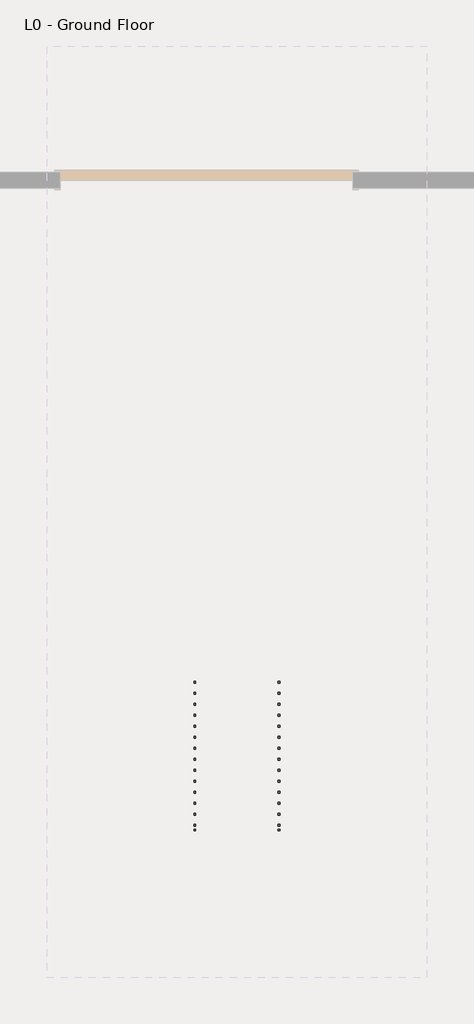
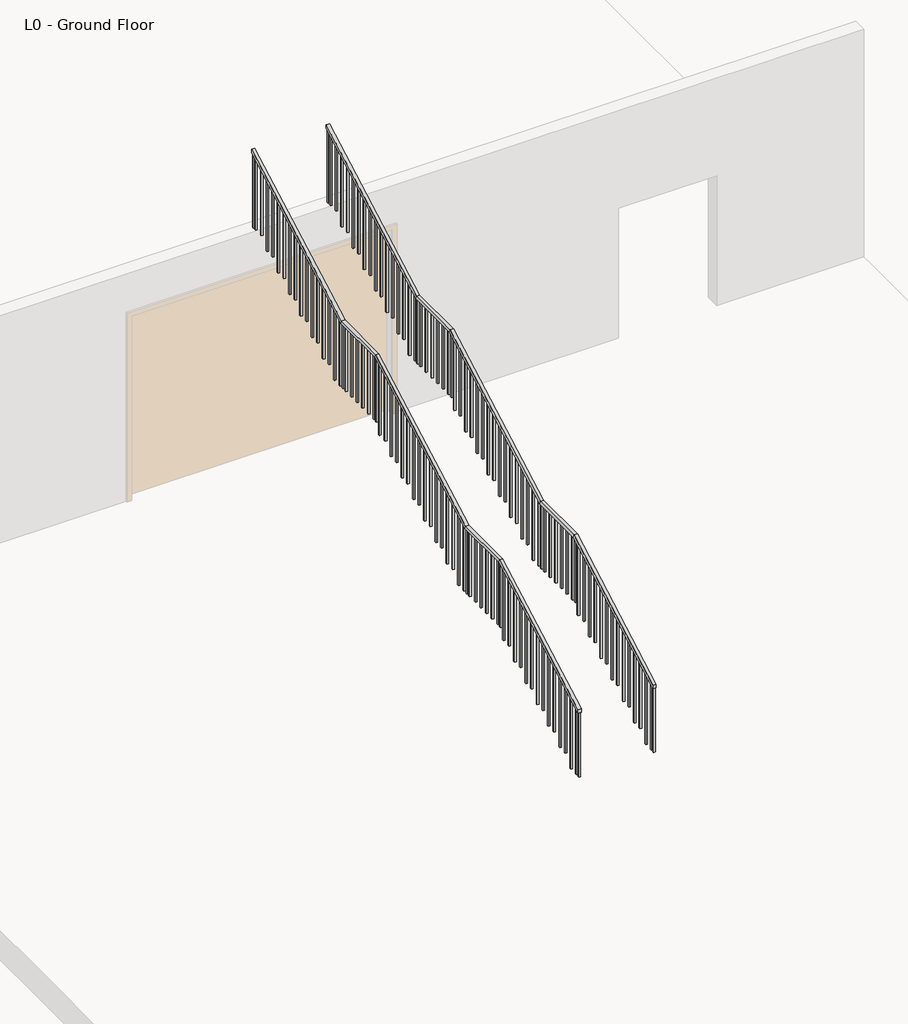
# One storey, part 10 of 14: 2 railings.
"""IFC4 building model written with IfcOpenShell, lengths in millimetres."""

from ifc_helpers import new_model, si_unit, frame, origin, place, context, project, spatial, polyline, outline, extrude, faceted_brep, element, save

model = new_model("IFC4")

# Units and contexts
model_context = context("Model", 3, world=origin())
ifc_project = project(units=[si_unit("LENGTHUNIT", "METRE", prefix="MILLI")], contexts=[model_context])

# Site, building, storey
site = spatial("IfcSite", under=ifc_project)
building = spatial("IfcBuilding", under=site)
storey = spatial("IfcBuildingStorey", under=building, Name="L0 - Ground Floor", Elevation=0.0)

# Railings
placement = place(None, origin())
element("IfcRailing", 1, ObjectType="1100mm", at=placement, inside=storey, context=model_context, shape_type="SolidModel", body=[
    faceted_brep([(20443.6510627, -13941.7341454, 1266.6666667), (20443.6510627, -13941.7341454, 1209.4687214), (20493.6510627, -13941.7341454, 1209.4687214), (20493.6510627, -13941.7341454, 1266.6666667), (20443.6510627, -11841.7341454, 2433.3333333), (20443.6510627, -11828.7778439, 2383.3333333), (20493.6510627, -11828.7778439, 2383.3333333), (20493.6510627, -11841.7341454, 2433.3333333), (20443.6510627, -10941.7341454, 2433.3333333), (20443.6510627, -10928.7778439, 2383.3333333), (20493.6510627, -10928.7778439, 2383.3333333), (20493.6510627, -10941.7341454, 2433.3333333), (20443.6510627, -8541.7341454, 3766.6666667), (20443.6510627, -8528.7778439, 3716.6666667), (20493.6510627, -8528.7778439, 3716.6666667), (20493.6510627, -8541.7341454, 3766.6666667), (20443.6510627, -7641.7341454, 3766.6666667), (20443.6510627, -7628.7778439, 3716.6666667), (20493.6510627, -7628.7778439, 3716.6666667), (20493.6510627, -7641.7341454, 3766.6666667), (20443.6510627, -5241.7341454, 5100.0), (20493.6510627, -5241.7341454, 5100.0), (20493.6510627, -5241.7341454, 5042.8020548), (20443.6510627, -5241.7341454, 5042.8020548)], [[[0, 1, 2, 3]], [[1, 0, 4, 5]], [[2, 1, 5, 6]], [[3, 2, 6, 7]], [[0, 3, 7, 4]], [[5, 4, 8, 9]], [[6, 5, 9, 10]], [[7, 6, 10, 11]], [[4, 7, 11, 8]], [[9, 8, 12, 13]], [[10, 9, 13, 14]], [[11, 10, 14, 15]], [[8, 11, 15, 12]], [[13, 12, 16, 17]], [[14, 13, 17, 18]], [[15, 14, 18, 19]], [[12, 15, 19, 16]], [[20, 21, 22, 23]], [[17, 16, 20, 23]], [[18, 17, 23, 22]], [[19, 18, 22, 21]], [[16, 19, 21, 20]]]),
    extrude(outline(polyline([(-5329.2341454, 3833.3333333), (-5329.2341454, 4994.1909437), (-5304.2341454, 5008.0798326), (-5304.2341454, 3833.3333333), (-5329.2341454, 3833.3333333)])), frame((20456.1510627, 0.0, 0.0), z_axis=(1.0, 0.0, 0.0), x_axis=(0.0, 1.0, 0.0)), (0.0, 0.0, 1.0), 25.0),
    extrude(outline(polyline([(-5479.2341454, 3833.3333333), (-5479.2341454, 4910.8576103), (-5454.2341454, 4924.7464992), (-5454.2341454, 3833.3333333), (-5479.2341454, 3833.3333333)])), frame((20456.1510627, 0.0, 0.0), z_axis=(1.0, 0.0, 0.0), x_axis=(0.0, 1.0, 0.0)), (0.0, 0.0, 1.0), 25.0),
    extrude(outline(polyline([(-5629.2341454, 3666.6666667), (-5629.2341454, 4827.524277), (-5604.2341454, 4841.4131659), (-5604.2341454, 3666.6666667), (-5629.2341454, 3666.6666667)])), frame((20456.1510627, 0.0, 0.0), z_axis=(1.0, 0.0, 0.0), x_axis=(0.0, 1.0, 0.0)), (0.0, 0.0, 1.0), 25.0),
    extrude(outline(polyline([(-5779.2341454, 3666.6666667), (-5779.2341454, 4744.1909437), (-5754.2341454, 4758.0798326), (-5754.2341454, 3666.6666667), (-5779.2341454, 3666.6666667)])), frame((20456.1510627, 0.0, 0.0), z_axis=(1.0, 0.0, 0.0), x_axis=(0.0, 1.0, 0.0)), (0.0, 0.0, 1.0), 25.0),
    extrude(outline(polyline([(-5929.2341454, 3500.0), (-5929.2341454, 4660.8576103), (-5904.2341454, 4674.7464992), (-5904.2341454, 3500.0), (-5929.2341454, 3500.0)])), frame((20456.1510627, 0.0, 0.0), z_axis=(1.0, 0.0, 0.0), x_axis=(0.0, 1.0, 0.0)), (0.0, 0.0, 1.0), 25.0),
    extrude(outline(polyline([(-6079.2341454, 3500.0), (-6079.2341454, 4577.524277), (-6054.2341454, 4591.4131659), (-6054.2341454, 3500.0), (-6079.2341454, 3500.0)])), frame((20456.1510627, 0.0, 0.0), z_axis=(1.0, 0.0, 0.0), x_axis=(0.0, 1.0, 0.0)), (0.0, 0.0, 1.0), 25.0),
    extrude(outline(polyline([(-6229.2341454, 3333.3333333), (-6229.2341454, 4494.1909437), (-6204.2341454, 4508.0798326), (-6204.2341454, 3333.3333333), (-6229.2341454, 3333.3333333)])), frame((20456.1510627, 0.0, 0.0), z_axis=(1.0, 0.0, 0.0), x_axis=(0.0, 1.0, 0.0)), (0.0, 0.0, 1.0), 25.0),
    extrude(outline(polyline([(-6379.2341454, 3333.3333333), (-6379.2341454, 4410.8576103), (-6354.2341454, 4424.7464992), (-6354.2341454, 3333.3333333), (-6379.2341454, 3333.3333333)])), frame((20456.1510627, 0.0, 0.0), z_axis=(1.0, 0.0, 0.0), x_axis=(0.0, 1.0, 0.0)), (0.0, 0.0, 1.0), 25.0),
    extrude(outline(polyline([(-6529.2341454, 3166.6666667), (-6529.2341454, 4327.524277), (-6504.2341454, 4341.4131659), (-6504.2341454, 3166.6666667), (-6529.2341454, 3166.6666667)])), frame((20456.1510627, 0.0, 0.0), z_axis=(1.0, 0.0, 0.0), x_axis=(0.0, 1.0, 0.0)), (0.0, 0.0, 1.0), 25.0),
    extrude(outline(polyline([(-6679.2341454, 3166.6666667), (-6679.2341454, 4244.1909437), (-6654.2341454, 4258.0798326), (-6654.2341454, 3166.6666667), (-6679.2341454, 3166.6666667)])), frame((20456.1510627, 0.0, 0.0), z_axis=(1.0, 0.0, 0.0), x_axis=(0.0, 1.0, 0.0)), (0.0, 0.0, 1.0), 25.0),
    extrude(outline(polyline([(-6829.2341454, 3000.0), (-6829.2341454, 4160.8576103), (-6804.2341454, 4174.7464992), (-6804.2341454, 3000.0), (-6829.2341454, 3000.0)])), frame((20456.1510627, 0.0, 0.0), z_axis=(1.0, 0.0, 0.0), x_axis=(0.0, 1.0, 0.0)), (0.0, 0.0, 1.0), 25.0),
    extrude(outline(polyline([(-6979.2341454, 3000.0), (-6979.2341454, 4077.524277), (-6954.2341454, 4091.4131659), (-6954.2341454, 3000.0), (-6979.2341454, 3000.0)])), frame((20456.1510627, 0.0, 0.0), z_axis=(1.0, 0.0, 0.0), x_axis=(0.0, 1.0, 0.0)), (0.0, 0.0, 1.0), 25.0),
    extrude(outline(polyline([(-7129.2341454, 2833.3333333), (-7129.2341454, 3994.1909437), (-7104.2341454, 4008.0798326), (-7104.2341454, 2833.3333333), (-7129.2341454, 2833.3333333)])), frame((20456.1510627, 0.0, 0.0), z_axis=(1.0, 0.0, 0.0), x_axis=(0.0, 1.0, 0.0)), (0.0, 0.0, 1.0), 25.0),
    extrude(outline(polyline([(-7279.2341454, 2833.3333333), (-7279.2341454, 3910.8576103), (-7254.2341454, 3924.7464992), (-7254.2341454, 2833.3333333), (-7279.2341454, 2833.3333333)])), frame((20456.1510627, 0.0, 0.0), z_axis=(1.0, 0.0, 0.0), x_axis=(0.0, 1.0, 0.0)), (0.0, 0.0, 1.0), 25.0),
    extrude(outline(polyline([(-7429.2341454, 2666.6666667), (-7429.2341454, 3827.524277), (-7404.2341454, 3841.4131659), (-7404.2341454, 2666.6666667), (-7429.2341454, 2666.6666667)])), frame((20456.1510627, 0.0, 0.0), z_axis=(1.0, 0.0, 0.0), x_axis=(0.0, 1.0, 0.0)), (0.0, 0.0, 1.0), 25.0),
    extrude(outline(polyline([(-7579.2341454, 2666.6666667), (-7579.2341454, 3744.1909437), (-7554.2341454, 3758.0798326), (-7554.2341454, 2666.6666667), (-7579.2341454, 2666.6666667)])), frame((20456.1510627, 0.0, 0.0), z_axis=(1.0, 0.0, 0.0), x_axis=(0.0, 1.0, 0.0)), (0.0, 0.0, 1.0), 25.0),
    extrude(outline(polyline([(20481.1510627, -7729.2341454), (20456.1510627, -7729.2341454), (20456.1510627, -7704.2341454), (20481.1510627, -7704.2341454), (20481.1510627, -7729.2341454)])), frame((0.0, 0.0, 2666.6666667), z_axis=(0.0, 0.0, 1.0), x_axis=(1.0, 0.0, 0.0)), (0.0, 0.0, 1.0), 1050.0),
    extrude(outline(polyline([(20481.1510627, -7879.2341454), (20456.1510627, -7879.2341454), (20456.1510627, -7854.2341454), (20481.1510627, -7854.2341454), (20481.1510627, -7879.2341454)])), frame((0.0, 0.0, 2666.6666667), z_axis=(0.0, 0.0, 1.0), x_axis=(1.0, 0.0, 0.0)), (0.0, 0.0, 1.0), 1050.0),
    extrude(outline(polyline([(20481.1510627, -8029.2341454), (20456.1510627, -8029.2341454), (20456.1510627, -8004.2341454), (20481.1510627, -8004.2341454), (20481.1510627, -8029.2341454)])), frame((0.0, 0.0, 2666.6666667), z_axis=(0.0, 0.0, 1.0), x_axis=(1.0, 0.0, 0.0)), (0.0, 0.0, 1.0), 1050.0),
    extrude(outline(polyline([(20481.1510627, -8179.2341454), (20456.1510627, -8179.2341454), (20456.1510627, -8154.2341454), (20481.1510627, -8154.2341454), (20481.1510627, -8179.2341454)])), frame((0.0, 0.0, 2666.6666667), z_axis=(0.0, 0.0, 1.0), x_axis=(1.0, 0.0, 0.0)), (0.0, 0.0, 1.0), 1050.0),
    extrude(outline(polyline([(20481.1510627, -8329.2341454), (20456.1510627, -8329.2341454), (20456.1510627, -8304.2341454), (20481.1510627, -8304.2341454), (20481.1510627, -8329.2341454)])), frame((0.0, 0.0, 2666.6666667), z_axis=(0.0, 0.0, 1.0), x_axis=(1.0, 0.0, 0.0)), (0.0, 0.0, 1.0), 1050.0),
    extrude(outline(polyline([(20481.1510627, -8479.2341454), (20456.1510627, -8479.2341454), (20456.1510627, -8454.2341454), (20481.1510627, -8454.2341454), (20481.1510627, -8479.2341454)])), frame((0.0, 0.0, 2666.6666667), z_axis=(0.0, 0.0, 1.0), x_axis=(1.0, 0.0, 0.0)), (0.0, 0.0, 1.0), 1050.0),
    extrude(outline(polyline([(-8629.2341454, 2500.0), (-8629.2341454, 3660.8576103), (-8604.2341454, 3674.7464992), (-8604.2341454, 2500.0), (-8629.2341454, 2500.0)])), frame((20456.1510627, 0.0, 0.0), z_axis=(1.0, 0.0, 0.0), x_axis=(0.0, 1.0, 0.0)), (0.0, 0.0, 1.0), 25.0),
    extrude(outline(polyline([(-8779.2341454, 2500.0), (-8779.2341454, 3577.524277), (-8754.2341454, 3591.4131659), (-8754.2341454, 2500.0), (-8779.2341454, 2500.0)])), frame((20456.1510627, 0.0, 0.0), z_axis=(1.0, 0.0, 0.0), x_axis=(0.0, 1.0, 0.0)), (0.0, 0.0, 1.0), 25.0),
    extrude(outline(polyline([(-8929.2341454, 2333.3333333), (-8929.2341454, 3494.1909437), (-8904.2341454, 3508.0798326), (-8904.2341454, 2333.3333333), (-8929.2341454, 2333.3333333)])), frame((20456.1510627, 0.0, 0.0), z_axis=(1.0, 0.0, 0.0), x_axis=(0.0, 1.0, 0.0)), (0.0, 0.0, 1.0), 25.0),
    extrude(outline(polyline([(-9079.2341454, 2333.3333333), (-9079.2341454, 3410.8576103), (-9054.2341454, 3424.7464992), (-9054.2341454, 2333.3333333), (-9079.2341454, 2333.3333333)])), frame((20456.1510627, 0.0, 0.0), z_axis=(1.0, 0.0, 0.0), x_axis=(0.0, 1.0, 0.0)), (0.0, 0.0, 1.0), 25.0),
    extrude(outline(polyline([(-9229.2341454, 2166.6666667), (-9229.2341454, 3327.524277), (-9204.2341454, 3341.4131659), (-9204.2341454, 2166.6666667), (-9229.2341454, 2166.6666667)])), frame((20456.1510627, 0.0, 0.0), z_axis=(1.0, 0.0, 0.0), x_axis=(0.0, 1.0, 0.0)), (0.0, 0.0, 1.0), 25.0),
    extrude(outline(polyline([(-9379.2341454, 2166.6666667), (-9379.2341454, 3244.1909437), (-9354.2341454, 3258.0798326), (-9354.2341454, 2166.6666667), (-9379.2341454, 2166.6666667)])), frame((20456.1510627, 0.0, 0.0), z_axis=(1.0, 0.0, 0.0), x_axis=(0.0, 1.0, 0.0)), (0.0, 0.0, 1.0), 25.0),
    extrude(outline(polyline([(-9529.2341454, 2000.0), (-9529.2341454, 3160.8576103), (-9504.2341454, 3174.7464992), (-9504.2341454, 2000.0), (-9529.2341454, 2000.0)])), frame((20456.1510627, 0.0, 0.0), z_axis=(1.0, 0.0, 0.0), x_axis=(0.0, 1.0, 0.0)), (0.0, 0.0, 1.0), 25.0),
    extrude(outline(polyline([(-9679.2341454, 2000.0), (-9679.2341454, 3077.524277), (-9654.2341454, 3091.4131659), (-9654.2341454, 2000.0), (-9679.2341454, 2000.0)])), frame((20456.1510627, 0.0, 0.0), z_axis=(1.0, 0.0, 0.0), x_axis=(0.0, 1.0, 0.0)), (0.0, 0.0, 1.0), 25.0),
    extrude(outline(polyline([(-9829.2341454, 1833.3333333), (-9829.2341454, 2994.1909437), (-9804.2341454, 3008.0798326), (-9804.2341454, 1833.3333333), (-9829.2341454, 1833.3333333)])), frame((20456.1510627, 0.0, 0.0), z_axis=(1.0, 0.0, 0.0), x_axis=(0.0, 1.0, 0.0)), (0.0, 0.0, 1.0), 25.0),
    extrude(outline(polyline([(-9979.2341454, 1833.3333333), (-9979.2341454, 2910.8576103), (-9954.2341454, 2924.7464992), (-9954.2341454, 1833.3333333), (-9979.2341454, 1833.3333333)])), frame((20456.1510627, 0.0, 0.0), z_axis=(1.0, 0.0, 0.0), x_axis=(0.0, 1.0, 0.0)), (0.0, 0.0, 1.0), 25.0),
    extrude(outline(polyline([(-10129.2341454, 1666.6666667), (-10129.2341454, 2827.524277), (-10104.2341454, 2841.4131659), (-10104.2341454, 1666.6666667), (-10129.2341454, 1666.6666667)])), frame((20456.1510627, 0.0, 0.0), z_axis=(1.0, 0.0, 0.0), x_axis=(0.0, 1.0, 0.0)), (0.0, 0.0, 1.0), 25.0),
    extrude(outline(polyline([(-10279.2341454, 1666.6666667), (-10279.2341454, 2744.1909437), (-10254.2341454, 2758.0798326), (-10254.2341454, 1666.6666667), (-10279.2341454, 1666.6666667)])), frame((20456.1510627, 0.0, 0.0), z_axis=(1.0, 0.0, 0.0), x_axis=(0.0, 1.0, 0.0)), (0.0, 0.0, 1.0), 25.0),
    extrude(outline(polyline([(-10429.2341454, 1500.0), (-10429.2341454, 2660.8576103), (-10404.2341454, 2674.7464992), (-10404.2341454, 1500.0), (-10429.2341454, 1500.0)])), frame((20456.1510627, 0.0, 0.0), z_axis=(1.0, 0.0, 0.0), x_axis=(0.0, 1.0, 0.0)), (0.0, 0.0, 1.0), 25.0),
    extrude(outline(polyline([(-10579.2341454, 1500.0), (-10579.2341454, 2577.524277), (-10554.2341454, 2591.4131659), (-10554.2341454, 1500.0), (-10579.2341454, 1500.0)])), frame((20456.1510627, 0.0, 0.0), z_axis=(1.0, 0.0, 0.0), x_axis=(0.0, 1.0, 0.0)), (0.0, 0.0, 1.0), 25.0),
    extrude(outline(polyline([(-10729.2341454, 1333.3333333), (-10729.2341454, 2494.1909437), (-10704.2341454, 2508.0798326), (-10704.2341454, 1333.3333333), (-10729.2341454, 1333.3333333)])), frame((20456.1510627, 0.0, 0.0), z_axis=(1.0, 0.0, 0.0), x_axis=(0.0, 1.0, 0.0)), (0.0, 0.0, 1.0), 25.0),
    extrude(outline(polyline([(-10879.2341454, 1333.3333333), (-10879.2341454, 2410.8576103), (-10854.2341454, 2424.7464992), (-10854.2341454, 1333.3333333), (-10879.2341454, 1333.3333333)])), frame((20456.1510627, 0.0, 0.0), z_axis=(1.0, 0.0, 0.0), x_axis=(0.0, 1.0, 0.0)), (0.0, 0.0, 1.0), 25.0),
    extrude(outline(polyline([(20481.1510627, -11029.2341454), (20456.1510627, -11029.2341454), (20456.1510627, -11004.2341454), (20481.1510627, -11004.2341454), (20481.1510627, -11029.2341454)])), frame((0.0, 0.0, 1333.3333333), z_axis=(0.0, 0.0, 1.0), x_axis=(1.0, 0.0, 0.0)), (0.0, 0.0, 1.0), 1050.0),
    extrude(outline(polyline([(20481.1510627, -11179.2341454), (20456.1510627, -11179.2341454), (20456.1510627, -11154.2341454), (20481.1510627, -11154.2341454), (20481.1510627, -11179.2341454)])), frame((0.0, 0.0, 1333.3333333), z_axis=(0.0, 0.0, 1.0), x_axis=(1.0, 0.0, 0.0)), (0.0, 0.0, 1.0), 1050.0),
    extrude(outline(polyline([(20481.1510627, -11329.2341454), (20456.1510627, -11329.2341454), (20456.1510627, -11304.2341454), (20481.1510627, -11304.2341454), (20481.1510627, -11329.2341454)])), frame((0.0, 0.0, 1333.3333333), z_axis=(0.0, 0.0, 1.0), x_axis=(1.0, 0.0, 0.0)), (0.0, 0.0, 1.0), 1050.0),
    extrude(outline(polyline([(20481.1510627, -11479.2341454), (20456.1510627, -11479.2341454), (20456.1510627, -11454.2341454), (20481.1510627, -11454.2341454), (20481.1510627, -11479.2341454)])), frame((0.0, 0.0, 1333.3333333), z_axis=(0.0, 0.0, 1.0), x_axis=(1.0, 0.0, 0.0)), (0.0, 0.0, 1.0), 1050.0),
    extrude(outline(polyline([(20481.1510627, -11629.2341454), (20456.1510627, -11629.2341454), (20456.1510627, -11604.2341454), (20481.1510627, -11604.2341454), (20481.1510627, -11629.2341454)])), frame((0.0, 0.0, 1333.3333333), z_axis=(0.0, 0.0, 1.0), x_axis=(1.0, 0.0, 0.0)), (0.0, 0.0, 1.0), 1050.0),
    extrude(outline(polyline([(20481.1510627, -11779.2341454), (20456.1510627, -11779.2341454), (20456.1510627, -11754.2341454), (20481.1510627, -11754.2341454), (20481.1510627, -11779.2341454)])), frame((0.0, 0.0, 1333.3333333), z_axis=(0.0, 0.0, 1.0), x_axis=(1.0, 0.0, 0.0)), (0.0, 0.0, 1.0), 1050.0),
    extrude(outline(polyline([(-11929.2341454, 1166.6666667), (-11929.2341454, 2327.524277), (-11904.2341454, 2341.4131659), (-11904.2341454, 1166.6666667), (-11929.2341454, 1166.6666667)])), frame((20456.1510627, 0.0, 0.0), z_axis=(1.0, 0.0, 0.0), x_axis=(0.0, 1.0, 0.0)), (0.0, 0.0, 1.0), 25.0),
    extrude(outline(polyline([(-12079.2341454, 1166.6666667), (-12079.2341454, 2244.1909437), (-12054.2341454, 2258.0798326), (-12054.2341454, 1166.6666667), (-12079.2341454, 1166.6666667)])), frame((20456.1510627, 0.0, 0.0), z_axis=(1.0, 0.0, 0.0), x_axis=(0.0, 1.0, 0.0)), (0.0, 0.0, 1.0), 25.0),
    extrude(outline(polyline([(-12229.2341454, 1000.0), (-12229.2341454, 2160.8576103), (-12204.2341454, 2174.7464992), (-12204.2341454, 1000.0), (-12229.2341454, 1000.0)])), frame((20456.1510627, 0.0, 0.0), z_axis=(1.0, 0.0, 0.0), x_axis=(0.0, 1.0, 0.0)), (0.0, 0.0, 1.0), 25.0),
    extrude(outline(polyline([(-12379.2341454, 1000.0), (-12379.2341454, 2077.524277), (-12354.2341454, 2091.4131659), (-12354.2341454, 1000.0), (-12379.2341454, 1000.0)])), frame((20456.1510627, 0.0, 0.0), z_axis=(1.0, 0.0, 0.0), x_axis=(0.0, 1.0, 0.0)), (0.0, 0.0, 1.0), 25.0),
    extrude(outline(polyline([(-12529.2341454, 833.3333333), (-12529.2341454, 1994.1909437), (-12504.2341454, 2008.0798326), (-12504.2341454, 833.3333333), (-12529.2341454, 833.3333333)])), frame((20456.1510627, 0.0, 0.0), z_axis=(1.0, 0.0, 0.0), x_axis=(0.0, 1.0, 0.0)), (0.0, 0.0, 1.0), 25.0),
    extrude(outline(polyline([(-12679.2341454, 833.3333333), (-12679.2341454, 1910.8576103), (-12654.2341454, 1924.7464992), (-12654.2341454, 833.3333333), (-12679.2341454, 833.3333333)])), frame((20456.1510627, 0.0, 0.0), z_axis=(1.0, 0.0, 0.0), x_axis=(0.0, 1.0, 0.0)), (0.0, 0.0, 1.0), 25.0),
    extrude(outline(polyline([(-12829.2341454, 666.6666667), (-12829.2341454, 1827.524277), (-12804.2341454, 1841.4131659), (-12804.2341454, 666.6666667), (-12829.2341454, 666.6666667)])), frame((20456.1510627, 0.0, 0.0), z_axis=(1.0, 0.0, 0.0), x_axis=(0.0, 1.0, 0.0)), (0.0, 0.0, 1.0), 25.0),
    extrude(outline(polyline([(-12979.2341454, 666.6666667), (-12979.2341454, 1744.1909437), (-12954.2341454, 1758.0798326), (-12954.2341454, 666.6666667), (-12979.2341454, 666.6666667)])), frame((20456.1510627, 0.0, 0.0), z_axis=(1.0, 0.0, 0.0), x_axis=(0.0, 1.0, 0.0)), (0.0, 0.0, 1.0), 25.0),
    extrude(outline(polyline([(-13129.2341454, 500.0), (-13129.2341454, 1660.8576103), (-13104.2341454, 1674.7464992), (-13104.2341454, 500.0), (-13129.2341454, 500.0)])), frame((20456.1510627, 0.0, 0.0), z_axis=(1.0, 0.0, 0.0), x_axis=(0.0, 1.0, 0.0)), (0.0, 0.0, 1.0), 25.0),
    extrude(outline(polyline([(-13279.2341454, 500.0), (-13279.2341454, 1577.524277), (-13254.2341454, 1591.4131659), (-13254.2341454, 500.0), (-13279.2341454, 500.0)])), frame((20456.1510627, 0.0, 0.0), z_axis=(1.0, 0.0, 0.0), x_axis=(0.0, 1.0, 0.0)), (0.0, 0.0, 1.0), 25.0),
    extrude(outline(polyline([(-13429.2341454, 333.3333333), (-13429.2341454, 1494.1909437), (-13404.2341454, 1508.0798326), (-13404.2341454, 333.3333333), (-13429.2341454, 333.3333333)])), frame((20456.1510627, 0.0, 0.0), z_axis=(1.0, 0.0, 0.0), x_axis=(0.0, 1.0, 0.0)), (0.0, 0.0, 1.0), 25.0),
    extrude(outline(polyline([(-13579.2341454, 333.3333333), (-13579.2341454, 1410.8576103), (-13554.2341454, 1424.7464992), (-13554.2341454, 333.3333333), (-13579.2341454, 333.3333333)])), frame((20456.1510627, 0.0, 0.0), z_axis=(1.0, 0.0, 0.0), x_axis=(0.0, 1.0, 0.0)), (0.0, 0.0, 1.0), 25.0),
    extrude(outline(polyline([(-13729.2341454, 166.6666667), (-13729.2341454, 1327.524277), (-13704.2341454, 1341.4131659), (-13704.2341454, 166.6666667), (-13729.2341454, 166.6666667)])), frame((20456.1510627, 0.0, 0.0), z_axis=(1.0, 0.0, 0.0), x_axis=(0.0, 1.0, 0.0)), (0.0, 0.0, 1.0), 25.0),
    extrude(outline(polyline([(-13879.2341454, 166.6666667), (-13879.2341454, 1244.1909437), (-13854.2341454, 1258.0798326), (-13854.2341454, 166.6666667), (-13879.2341454, 166.6666667)])), frame((20456.1510627, 0.0, 0.0), z_axis=(1.0, 0.0, 0.0), x_axis=(0.0, 1.0, 0.0)), (0.0, 0.0, 1.0), 25.0),
    extrude(outline(polyline([(20481.1510627, -7654.2341454), (20456.1510627, -7654.2341454), (20456.1510627, -7629.2341454), (20481.1510627, -7629.2341454), (20481.1510627, -7654.2341454)])), frame((0.0, 0.0, 2666.6666667), z_axis=(0.0, 0.0, 1.0), x_axis=(1.0, 0.0, 0.0)), (0.0, 0.0, 1.0), 1050.0),
    extrude(outline(polyline([(-8554.2341454, 2666.6666667), (-8554.2341454, 3702.524277), (-8529.2341454, 3716.4131659), (-8529.2341454, 2666.6666667), (-8554.2341454, 2666.6666667)])), frame((20456.1510627, 0.0, 0.0), z_axis=(1.0, 0.0, 0.0), x_axis=(0.0, 1.0, 0.0)), (0.0, 0.0, 1.0), 25.0),
    extrude(outline(polyline([(20481.1510627, -10954.2341454), (20456.1510627, -10954.2341454), (20456.1510627, -10929.2341454), (20481.1510627, -10929.2341454), (20481.1510627, -10954.2341454)])), frame((0.0, 0.0, 1333.3333333), z_axis=(0.0, 0.0, 1.0), x_axis=(1.0, 0.0, 0.0)), (0.0, 0.0, 1.0), 1050.0),
    extrude(outline(polyline([(-11854.2341454, 1333.3333333), (-11854.2341454, 2369.1909437), (-11829.2341454, 2383.0798326), (-11829.2341454, 1333.3333333), (-11854.2341454, 1333.3333333)])), frame((20456.1510627, 0.0, 0.0), z_axis=(1.0, 0.0, 0.0), x_axis=(0.0, 1.0, 0.0)), (0.0, 0.0, 1.0), 25.0),
    extrude(outline(polyline([(-5266.7341454, 3833.3333333), (-5266.7341454, 5028.9131659), (-5241.7341454, 5042.8020548), (-5241.7341454, 3833.3333333), (-5266.7341454, 3833.3333333)])), frame((20456.1510627, 0.0, 0.0), z_axis=(1.0, 0.0, 0.0), x_axis=(0.0, 1.0, 0.0)), (0.0, 0.0, 1.0), 25.0),
    extrude(outline(polyline([(-13941.7341454, 166.6666667), (-13941.7341454, 1209.4687214), (-13916.7341454, 1223.3576103), (-13916.7341454, 166.6666667), (-13941.7341454, 166.6666667)])), frame((20456.1510627, 0.0, 0.0), z_axis=(1.0, 0.0, 0.0), x_axis=(0.0, 1.0, 0.0)), (0.0, 0.0, 1.0), 25.0),
])
element("IfcRailing", 2, ObjectType="1100mm", at=placement, inside=storey, context=model_context, shape_type="SolidModel", body=[
    faceted_brep([(19294.4510627, -13941.7341454, 1266.6666667), (19294.4510627, -13941.7341454, 1209.4687214), (19344.4510627, -13941.7341454, 1209.4687214), (19344.4510627, -13941.7341454, 1266.6666667), (19294.4510627, -11841.7341454, 2433.3333333), (19294.4510627, -11828.7778439, 2383.3333333), (19344.4510627, -11828.7778439, 2383.3333333), (19344.4510627, -11841.7341454, 2433.3333333), (19294.4510627, -10941.7341454, 2433.3333333), (19294.4510627, -10928.7778439, 2383.3333333), (19344.4510627, -10928.7778439, 2383.3333333), (19344.4510627, -10941.7341454, 2433.3333333), (19294.4510627, -8541.7341454, 3766.6666667), (19294.4510627, -8528.7778439, 3716.6666667), (19344.4510627, -8528.7778439, 3716.6666667), (19344.4510627, -8541.7341454, 3766.6666667), (19294.4510627, -7641.7341454, 3766.6666667), (19294.4510627, -7628.7778439, 3716.6666667), (19344.4510627, -7628.7778439, 3716.6666667), (19344.4510627, -7641.7341454, 3766.6666667), (19294.4510627, -5241.7341454, 5100.0), (19344.4510627, -5241.7341454, 5100.0), (19344.4510627, -5241.7341454, 5042.8020548), (19294.4510627, -5241.7341454, 5042.8020548)], [[[0, 1, 2, 3]], [[1, 0, 4, 5]], [[2, 1, 5, 6]], [[3, 2, 6, 7]], [[0, 3, 7, 4]], [[5, 4, 8, 9]], [[6, 5, 9, 10]], [[7, 6, 10, 11]], [[4, 7, 11, 8]], [[9, 8, 12, 13]], [[10, 9, 13, 14]], [[11, 10, 14, 15]], [[8, 11, 15, 12]], [[13, 12, 16, 17]], [[14, 13, 17, 18]], [[15, 14, 18, 19]], [[12, 15, 19, 16]], [[20, 21, 22, 23]], [[17, 16, 20, 23]], [[18, 17, 23, 22]], [[19, 18, 22, 21]], [[16, 19, 21, 20]]]),
    extrude(outline(polyline([(-5329.2341454, 4994.1909437), (-5304.2341454, 5008.0798326), (-5304.2341454, 3833.3333333), (-5329.2341454, 3833.3333333), (-5329.2341454, 4994.1909437)])), frame((19306.9510627, 0.0, 0.0), z_axis=(1.0, 0.0, 0.0), x_axis=(0.0, 1.0, 0.0)), (0.0, 0.0, 1.0), 25.0),
    extrude(outline(polyline([(-5479.2341454, 4910.8576103), (-5454.2341454, 4924.7464992), (-5454.2341454, 3833.3333333), (-5479.2341454, 3833.3333333), (-5479.2341454, 4910.8576103)])), frame((19306.9510627, 0.0, 0.0), z_axis=(1.0, 0.0, 0.0), x_axis=(0.0, 1.0, 0.0)), (0.0, 0.0, 1.0), 25.0),
    extrude(outline(polyline([(-5629.2341454, 4827.524277), (-5604.2341454, 4841.4131659), (-5604.2341454, 3666.6666667), (-5629.2341454, 3666.6666667), (-5629.2341454, 4827.524277)])), frame((19306.9510627, 0.0, 0.0), z_axis=(1.0, 0.0, 0.0), x_axis=(0.0, 1.0, 0.0)), (0.0, 0.0, 1.0), 25.0),
    extrude(outline(polyline([(-5779.2341454, 4744.1909437), (-5754.2341454, 4758.0798326), (-5754.2341454, 3666.6666667), (-5779.2341454, 3666.6666667), (-5779.2341454, 4744.1909437)])), frame((19306.9510627, 0.0, 0.0), z_axis=(1.0, 0.0, 0.0), x_axis=(0.0, 1.0, 0.0)), (0.0, 0.0, 1.0), 25.0),
    extrude(outline(polyline([(-5929.2341454, 4660.8576103), (-5904.2341454, 4674.7464992), (-5904.2341454, 3500.0), (-5929.2341454, 3500.0), (-5929.2341454, 4660.8576103)])), frame((19306.9510627, 0.0, 0.0), z_axis=(1.0, 0.0, 0.0), x_axis=(0.0, 1.0, 0.0)), (0.0, 0.0, 1.0), 25.0),
    extrude(outline(polyline([(-6079.2341454, 4577.524277), (-6054.2341454, 4591.4131659), (-6054.2341454, 3500.0), (-6079.2341454, 3500.0), (-6079.2341454, 4577.524277)])), frame((19306.9510627, 0.0, 0.0), z_axis=(1.0, 0.0, 0.0), x_axis=(0.0, 1.0, 0.0)), (0.0, 0.0, 1.0), 25.0),
    extrude(outline(polyline([(-6229.2341454, 4494.1909437), (-6204.2341454, 4508.0798326), (-6204.2341454, 3333.3333333), (-6229.2341454, 3333.3333333), (-6229.2341454, 4494.1909437)])), frame((19306.9510627, 0.0, 0.0), z_axis=(1.0, 0.0, 0.0), x_axis=(0.0, 1.0, 0.0)), (0.0, 0.0, 1.0), 25.0),
    extrude(outline(polyline([(-6379.2341454, 4410.8576103), (-6354.2341454, 4424.7464992), (-6354.2341454, 3333.3333333), (-6379.2341454, 3333.3333333), (-6379.2341454, 4410.8576103)])), frame((19306.9510627, 0.0, 0.0), z_axis=(1.0, 0.0, 0.0), x_axis=(0.0, 1.0, 0.0)), (0.0, 0.0, 1.0), 25.0),
    extrude(outline(polyline([(-6529.2341454, 4327.524277), (-6504.2341454, 4341.4131659), (-6504.2341454, 3166.6666667), (-6529.2341454, 3166.6666667), (-6529.2341454, 4327.524277)])), frame((19306.9510627, 0.0, 0.0), z_axis=(1.0, 0.0, 0.0), x_axis=(0.0, 1.0, 0.0)), (0.0, 0.0, 1.0), 25.0),
    extrude(outline(polyline([(-6679.2341454, 4244.1909437), (-6654.2341454, 4258.0798326), (-6654.2341454, 3166.6666667), (-6679.2341454, 3166.6666667), (-6679.2341454, 4244.1909437)])), frame((19306.9510627, 0.0, 0.0), z_axis=(1.0, 0.0, 0.0), x_axis=(0.0, 1.0, 0.0)), (0.0, 0.0, 1.0), 25.0),
    extrude(outline(polyline([(-6829.2341454, 4160.8576103), (-6804.2341454, 4174.7464992), (-6804.2341454, 3000.0), (-6829.2341454, 3000.0), (-6829.2341454, 4160.8576103)])), frame((19306.9510627, 0.0, 0.0), z_axis=(1.0, 0.0, 0.0), x_axis=(0.0, 1.0, 0.0)), (0.0, 0.0, 1.0), 25.0),
    extrude(outline(polyline([(-6979.2341454, 4077.524277), (-6954.2341454, 4091.4131659), (-6954.2341454, 3000.0), (-6979.2341454, 3000.0), (-6979.2341454, 4077.524277)])), frame((19306.9510627, 0.0, 0.0), z_axis=(1.0, 0.0, 0.0), x_axis=(0.0, 1.0, 0.0)), (0.0, 0.0, 1.0), 25.0),
    extrude(outline(polyline([(-7129.2341454, 3994.1909437), (-7104.2341454, 4008.0798326), (-7104.2341454, 2833.3333333), (-7129.2341454, 2833.3333333), (-7129.2341454, 3994.1909437)])), frame((19306.9510627, 0.0, 0.0), z_axis=(1.0, 0.0, 0.0), x_axis=(0.0, 1.0, 0.0)), (0.0, 0.0, 1.0), 25.0),
    extrude(outline(polyline([(-7279.2341454, 3910.8576103), (-7254.2341454, 3924.7464992), (-7254.2341454, 2833.3333333), (-7279.2341454, 2833.3333333), (-7279.2341454, 3910.8576103)])), frame((19306.9510627, 0.0, 0.0), z_axis=(1.0, 0.0, 0.0), x_axis=(0.0, 1.0, 0.0)), (0.0, 0.0, 1.0), 25.0),
    extrude(outline(polyline([(-7429.2341454, 3827.524277), (-7404.2341454, 3841.4131659), (-7404.2341454, 2666.6666667), (-7429.2341454, 2666.6666667), (-7429.2341454, 3827.524277)])), frame((19306.9510627, 0.0, 0.0), z_axis=(1.0, 0.0, 0.0), x_axis=(0.0, 1.0, 0.0)), (0.0, 0.0, 1.0), 25.0),
    extrude(outline(polyline([(-7579.2341454, 3744.1909437), (-7554.2341454, 3758.0798326), (-7554.2341454, 2666.6666667), (-7579.2341454, 2666.6666667), (-7579.2341454, 3744.1909437)])), frame((19306.9510627, 0.0, 0.0), z_axis=(1.0, 0.0, 0.0), x_axis=(0.0, 1.0, 0.0)), (0.0, 0.0, 1.0), 25.0),
    extrude(outline(polyline([(19306.9510627, -7729.2341454), (19306.9510627, -7704.2341454), (19331.9510627, -7704.2341454), (19331.9510627, -7729.2341454), (19306.9510627, -7729.2341454)])), frame((0.0, 0.0, 2666.6666667), z_axis=(0.0, 0.0, 1.0), x_axis=(1.0, 0.0, 0.0)), (0.0, 0.0, 1.0), 1050.0),
    extrude(outline(polyline([(19306.9510627, -7879.2341454), (19306.9510627, -7854.2341454), (19331.9510627, -7854.2341454), (19331.9510627, -7879.2341454), (19306.9510627, -7879.2341454)])), frame((0.0, 0.0, 2666.6666667), z_axis=(0.0, 0.0, 1.0), x_axis=(1.0, 0.0, 0.0)), (0.0, 0.0, 1.0), 1050.0),
    extrude(outline(polyline([(19306.9510627, -8029.2341454), (19306.9510627, -8004.2341454), (19331.9510627, -8004.2341454), (19331.9510627, -8029.2341454), (19306.9510627, -8029.2341454)])), frame((0.0, 0.0, 2666.6666667), z_axis=(0.0, 0.0, 1.0), x_axis=(1.0, 0.0, 0.0)), (0.0, 0.0, 1.0), 1050.0),
    extrude(outline(polyline([(19306.9510627, -8179.2341454), (19306.9510627, -8154.2341454), (19331.9510627, -8154.2341454), (19331.9510627, -8179.2341454), (19306.9510627, -8179.2341454)])), frame((0.0, 0.0, 2666.6666667), z_axis=(0.0, 0.0, 1.0), x_axis=(1.0, 0.0, 0.0)), (0.0, 0.0, 1.0), 1050.0),
    extrude(outline(polyline([(19306.9510627, -8329.2341454), (19306.9510627, -8304.2341454), (19331.9510627, -8304.2341454), (19331.9510627, -8329.2341454), (19306.9510627, -8329.2341454)])), frame((0.0, 0.0, 2666.6666667), z_axis=(0.0, 0.0, 1.0), x_axis=(1.0, 0.0, 0.0)), (0.0, 0.0, 1.0), 1050.0),
    extrude(outline(polyline([(19306.9510627, -8479.2341454), (19306.9510627, -8454.2341454), (19331.9510627, -8454.2341454), (19331.9510627, -8479.2341454), (19306.9510627, -8479.2341454)])), frame((0.0, 0.0, 2666.6666667), z_axis=(0.0, 0.0, 1.0), x_axis=(1.0, 0.0, 0.0)), (0.0, 0.0, 1.0), 1050.0),
    extrude(outline(polyline([(-8629.2341454, 3660.8576103), (-8604.2341454, 3674.7464992), (-8604.2341454, 2500.0), (-8629.2341454, 2500.0), (-8629.2341454, 3660.8576103)])), frame((19306.9510627, 0.0, 0.0), z_axis=(1.0, 0.0, 0.0), x_axis=(0.0, 1.0, 0.0)), (0.0, 0.0, 1.0), 25.0),
    extrude(outline(polyline([(-8779.2341454, 3577.524277), (-8754.2341454, 3591.4131659), (-8754.2341454, 2500.0), (-8779.2341454, 2500.0), (-8779.2341454, 3577.524277)])), frame((19306.9510627, 0.0, 0.0), z_axis=(1.0, 0.0, 0.0), x_axis=(0.0, 1.0, 0.0)), (0.0, 0.0, 1.0), 25.0),
    extrude(outline(polyline([(-8929.2341454, 3494.1909437), (-8904.2341454, 3508.0798326), (-8904.2341454, 2333.3333333), (-8929.2341454, 2333.3333333), (-8929.2341454, 3494.1909437)])), frame((19306.9510627, 0.0, 0.0), z_axis=(1.0, 0.0, 0.0), x_axis=(0.0, 1.0, 0.0)), (0.0, 0.0, 1.0), 25.0),
    extrude(outline(polyline([(-9079.2341454, 3410.8576103), (-9054.2341454, 3424.7464992), (-9054.2341454, 2333.3333333), (-9079.2341454, 2333.3333333), (-9079.2341454, 3410.8576103)])), frame((19306.9510627, 0.0, 0.0), z_axis=(1.0, 0.0, 0.0), x_axis=(0.0, 1.0, 0.0)), (0.0, 0.0, 1.0), 25.0),
    extrude(outline(polyline([(-9229.2341454, 3327.524277), (-9204.2341454, 3341.4131659), (-9204.2341454, 2166.6666667), (-9229.2341454, 2166.6666667), (-9229.2341454, 3327.524277)])), frame((19306.9510627, 0.0, 0.0), z_axis=(1.0, 0.0, 0.0), x_axis=(0.0, 1.0, 0.0)), (0.0, 0.0, 1.0), 25.0),
    extrude(outline(polyline([(-9379.2341454, 3244.1909437), (-9354.2341454, 3258.0798326), (-9354.2341454, 2166.6666667), (-9379.2341454, 2166.6666667), (-9379.2341454, 3244.1909437)])), frame((19306.9510627, 0.0, 0.0), z_axis=(1.0, 0.0, 0.0), x_axis=(0.0, 1.0, 0.0)), (0.0, 0.0, 1.0), 25.0),
    extrude(outline(polyline([(-9529.2341454, 3160.8576103), (-9504.2341454, 3174.7464992), (-9504.2341454, 2000.0), (-9529.2341454, 2000.0), (-9529.2341454, 3160.8576103)])), frame((19306.9510627, 0.0, 0.0), z_axis=(1.0, 0.0, 0.0), x_axis=(0.0, 1.0, 0.0)), (0.0, 0.0, 1.0), 25.0),
    extrude(outline(polyline([(-9679.2341454, 3077.524277), (-9654.2341454, 3091.4131659), (-9654.2341454, 2000.0), (-9679.2341454, 2000.0), (-9679.2341454, 3077.524277)])), frame((19306.9510627, 0.0, 0.0), z_axis=(1.0, 0.0, 0.0), x_axis=(0.0, 1.0, 0.0)), (0.0, 0.0, 1.0), 25.0),
    extrude(outline(polyline([(-9829.2341454, 2994.1909437), (-9804.2341454, 3008.0798326), (-9804.2341454, 1833.3333333), (-9829.2341454, 1833.3333333), (-9829.2341454, 2994.1909437)])), frame((19306.9510627, 0.0, 0.0), z_axis=(1.0, 0.0, 0.0), x_axis=(0.0, 1.0, 0.0)), (0.0, 0.0, 1.0), 25.0),
    extrude(outline(polyline([(-9979.2341454, 2910.8576103), (-9954.2341454, 2924.7464992), (-9954.2341454, 1833.3333333), (-9979.2341454, 1833.3333333), (-9979.2341454, 2910.8576103)])), frame((19306.9510627, 0.0, 0.0), z_axis=(1.0, 0.0, 0.0), x_axis=(0.0, 1.0, 0.0)), (0.0, 0.0, 1.0), 25.0),
    extrude(outline(polyline([(-10129.2341454, 2827.524277), (-10104.2341454, 2841.4131659), (-10104.2341454, 1666.6666667), (-10129.2341454, 1666.6666667), (-10129.2341454, 2827.524277)])), frame((19306.9510627, 0.0, 0.0), z_axis=(1.0, 0.0, 0.0), x_axis=(0.0, 1.0, 0.0)), (0.0, 0.0, 1.0), 25.0),
    extrude(outline(polyline([(-10279.2341454, 2744.1909437), (-10254.2341454, 2758.0798326), (-10254.2341454, 1666.6666667), (-10279.2341454, 1666.6666667), (-10279.2341454, 2744.1909437)])), frame((19306.9510627, 0.0, 0.0), z_axis=(1.0, 0.0, 0.0), x_axis=(0.0, 1.0, 0.0)), (0.0, 0.0, 1.0), 25.0),
    extrude(outline(polyline([(-10429.2341454, 2660.8576103), (-10404.2341454, 2674.7464992), (-10404.2341454, 1500.0), (-10429.2341454, 1500.0), (-10429.2341454, 2660.8576103)])), frame((19306.9510627, 0.0, 0.0), z_axis=(1.0, 0.0, 0.0), x_axis=(0.0, 1.0, 0.0)), (0.0, 0.0, 1.0), 25.0),
    extrude(outline(polyline([(-10579.2341454, 2577.524277), (-10554.2341454, 2591.4131659), (-10554.2341454, 1500.0), (-10579.2341454, 1500.0), (-10579.2341454, 2577.524277)])), frame((19306.9510627, 0.0, 0.0), z_axis=(1.0, 0.0, 0.0), x_axis=(0.0, 1.0, 0.0)), (0.0, 0.0, 1.0), 25.0),
    extrude(outline(polyline([(-10729.2341454, 2494.1909437), (-10704.2341454, 2508.0798326), (-10704.2341454, 1333.3333333), (-10729.2341454, 1333.3333333), (-10729.2341454, 2494.1909437)])), frame((19306.9510627, 0.0, 0.0), z_axis=(1.0, 0.0, 0.0), x_axis=(0.0, 1.0, 0.0)), (0.0, 0.0, 1.0), 25.0),
    extrude(outline(polyline([(-10879.2341454, 2410.8576103), (-10854.2341454, 2424.7464992), (-10854.2341454, 1333.3333333), (-10879.2341454, 1333.3333333), (-10879.2341454, 2410.8576103)])), frame((19306.9510627, 0.0, 0.0), z_axis=(1.0, 0.0, 0.0), x_axis=(0.0, 1.0, 0.0)), (0.0, 0.0, 1.0), 25.0),
    extrude(outline(polyline([(19306.9510627, -11029.2341454), (19306.9510627, -11004.2341454), (19331.9510627, -11004.2341454), (19331.9510627, -11029.2341454), (19306.9510627, -11029.2341454)])), frame((0.0, 0.0, 1333.3333333), z_axis=(0.0, 0.0, 1.0), x_axis=(1.0, 0.0, 0.0)), (0.0, 0.0, 1.0), 1050.0),
    extrude(outline(polyline([(19306.9510627, -11179.2341454), (19306.9510627, -11154.2341454), (19331.9510627, -11154.2341454), (19331.9510627, -11179.2341454), (19306.9510627, -11179.2341454)])), frame((0.0, 0.0, 1333.3333333), z_axis=(0.0, 0.0, 1.0), x_axis=(1.0, 0.0, 0.0)), (0.0, 0.0, 1.0), 1050.0),
    extrude(outline(polyline([(19306.9510627, -11329.2341454), (19306.9510627, -11304.2341454), (19331.9510627, -11304.2341454), (19331.9510627, -11329.2341454), (19306.9510627, -11329.2341454)])), frame((0.0, 0.0, 1333.3333333), z_axis=(0.0, 0.0, 1.0), x_axis=(1.0, 0.0, 0.0)), (0.0, 0.0, 1.0), 1050.0),
    extrude(outline(polyline([(19306.9510627, -11479.2341454), (19306.9510627, -11454.2341454), (19331.9510627, -11454.2341454), (19331.9510627, -11479.2341454), (19306.9510627, -11479.2341454)])), frame((0.0, 0.0, 1333.3333333), z_axis=(0.0, 0.0, 1.0), x_axis=(1.0, 0.0, 0.0)), (0.0, 0.0, 1.0), 1050.0),
    extrude(outline(polyline([(19306.9510627, -11629.2341454), (19306.9510627, -11604.2341454), (19331.9510627, -11604.2341454), (19331.9510627, -11629.2341454), (19306.9510627, -11629.2341454)])), frame((0.0, 0.0, 1333.3333333), z_axis=(0.0, 0.0, 1.0), x_axis=(1.0, 0.0, 0.0)), (0.0, 0.0, 1.0), 1050.0),
    extrude(outline(polyline([(19306.9510627, -11779.2341454), (19306.9510627, -11754.2341454), (19331.9510627, -11754.2341454), (19331.9510627, -11779.2341454), (19306.9510627, -11779.2341454)])), frame((0.0, 0.0, 1333.3333333), z_axis=(0.0, 0.0, 1.0), x_axis=(1.0, 0.0, 0.0)), (0.0, 0.0, 1.0), 1050.0),
    extrude(outline(polyline([(-11929.2341454, 2327.524277), (-11904.2341454, 2341.4131659), (-11904.2341454, 1166.6666667), (-11929.2341454, 1166.6666667), (-11929.2341454, 2327.524277)])), frame((19306.9510627, 0.0, 0.0), z_axis=(1.0, 0.0, 0.0), x_axis=(0.0, 1.0, 0.0)), (0.0, 0.0, 1.0), 25.0),
    extrude(outline(polyline([(-12079.2341454, 2244.1909437), (-12054.2341454, 2258.0798326), (-12054.2341454, 1166.6666667), (-12079.2341454, 1166.6666667), (-12079.2341454, 2244.1909437)])), frame((19306.9510627, 0.0, 0.0), z_axis=(1.0, 0.0, 0.0), x_axis=(0.0, 1.0, 0.0)), (0.0, 0.0, 1.0), 25.0),
    extrude(outline(polyline([(-12229.2341454, 2160.8576103), (-12204.2341454, 2174.7464992), (-12204.2341454, 1000.0), (-12229.2341454, 1000.0), (-12229.2341454, 2160.8576103)])), frame((19306.9510627, 0.0, 0.0), z_axis=(1.0, 0.0, 0.0), x_axis=(0.0, 1.0, 0.0)), (0.0, 0.0, 1.0), 25.0),
    extrude(outline(polyline([(-12379.2341454, 2077.524277), (-12354.2341454, 2091.4131659), (-12354.2341454, 1000.0), (-12379.2341454, 1000.0), (-12379.2341454, 2077.524277)])), frame((19306.9510627, 0.0, 0.0), z_axis=(1.0, 0.0, 0.0), x_axis=(0.0, 1.0, 0.0)), (0.0, 0.0, 1.0), 25.0),
    extrude(outline(polyline([(-12529.2341454, 1994.1909437), (-12504.2341454, 2008.0798326), (-12504.2341454, 833.3333333), (-12529.2341454, 833.3333333), (-12529.2341454, 1994.1909437)])), frame((19306.9510627, 0.0, 0.0), z_axis=(1.0, 0.0, 0.0), x_axis=(0.0, 1.0, 0.0)), (0.0, 0.0, 1.0), 25.0),
    extrude(outline(polyline([(-12679.2341454, 1910.8576103), (-12654.2341454, 1924.7464992), (-12654.2341454, 833.3333333), (-12679.2341454, 833.3333333), (-12679.2341454, 1910.8576103)])), frame((19306.9510627, 0.0, 0.0), z_axis=(1.0, 0.0, 0.0), x_axis=(0.0, 1.0, 0.0)), (0.0, 0.0, 1.0), 25.0),
    extrude(outline(polyline([(-12829.2341454, 1827.524277), (-12804.2341454, 1841.4131659), (-12804.2341454, 666.6666667), (-12829.2341454, 666.6666667), (-12829.2341454, 1827.524277)])), frame((19306.9510627, 0.0, 0.0), z_axis=(1.0, 0.0, 0.0), x_axis=(0.0, 1.0, 0.0)), (0.0, 0.0, 1.0), 25.0),
    extrude(outline(polyline([(-12979.2341454, 1744.1909437), (-12954.2341454, 1758.0798326), (-12954.2341454, 666.6666667), (-12979.2341454, 666.6666667), (-12979.2341454, 1744.1909437)])), frame((19306.9510627, 0.0, 0.0), z_axis=(1.0, 0.0, 0.0), x_axis=(0.0, 1.0, 0.0)), (0.0, 0.0, 1.0), 25.0),
    extrude(outline(polyline([(-13129.2341454, 1660.8576103), (-13104.2341454, 1674.7464992), (-13104.2341454, 500.0), (-13129.2341454, 500.0), (-13129.2341454, 1660.8576103)])), frame((19306.9510627, 0.0, 0.0), z_axis=(1.0, 0.0, 0.0), x_axis=(0.0, 1.0, 0.0)), (0.0, 0.0, 1.0), 25.0),
    extrude(outline(polyline([(-13279.2341454, 1577.524277), (-13254.2341454, 1591.4131659), (-13254.2341454, 500.0), (-13279.2341454, 500.0), (-13279.2341454, 1577.524277)])), frame((19306.9510627, 0.0, 0.0), z_axis=(1.0, 0.0, 0.0), x_axis=(0.0, 1.0, 0.0)), (0.0, 0.0, 1.0), 25.0),
    extrude(outline(polyline([(-13429.2341454, 1494.1909437), (-13404.2341454, 1508.0798326), (-13404.2341454, 333.3333333), (-13429.2341454, 333.3333333), (-13429.2341454, 1494.1909437)])), frame((19306.9510627, 0.0, 0.0), z_axis=(1.0, 0.0, 0.0), x_axis=(0.0, 1.0, 0.0)), (0.0, 0.0, 1.0), 25.0),
    extrude(outline(polyline([(-13579.2341454, 1410.8576103), (-13554.2341454, 1424.7464992), (-13554.2341454, 333.3333333), (-13579.2341454, 333.3333333), (-13579.2341454, 1410.8576103)])), frame((19306.9510627, 0.0, 0.0), z_axis=(1.0, 0.0, 0.0), x_axis=(0.0, 1.0, 0.0)), (0.0, 0.0, 1.0), 25.0),
    extrude(outline(polyline([(-13729.2341454, 1327.524277), (-13704.2341454, 1341.4131659), (-13704.2341454, 166.6666667), (-13729.2341454, 166.6666667), (-13729.2341454, 1327.524277)])), frame((19306.9510627, 0.0, 0.0), z_axis=(1.0, 0.0, 0.0), x_axis=(0.0, 1.0, 0.0)), (0.0, 0.0, 1.0), 25.0),
    extrude(outline(polyline([(-13879.2341454, 1244.1909437), (-13854.2341454, 1258.0798326), (-13854.2341454, 166.6666667), (-13879.2341454, 166.6666667), (-13879.2341454, 1244.1909437)])), frame((19306.9510627, 0.0, 0.0), z_axis=(1.0, 0.0, 0.0), x_axis=(0.0, 1.0, 0.0)), (0.0, 0.0, 1.0), 25.0),
    extrude(outline(polyline([(19306.9510627, -7654.2341454), (19306.9510627, -7629.2341454), (19331.9510627, -7629.2341454), (19331.9510627, -7654.2341454), (19306.9510627, -7654.2341454)])), frame((0.0, 0.0, 2666.6666667), z_axis=(0.0, 0.0, 1.0), x_axis=(1.0, 0.0, 0.0)), (0.0, 0.0, 1.0), 1050.0),
    extrude(outline(polyline([(-8554.2341454, 3702.524277), (-8529.2341454, 3716.4131659), (-8529.2341454, 2666.6666667), (-8554.2341454, 2666.6666667), (-8554.2341454, 3702.524277)])), frame((19306.9510627, 0.0, 0.0), z_axis=(1.0, 0.0, 0.0), x_axis=(0.0, 1.0, 0.0)), (0.0, 0.0, 1.0), 25.0),
    extrude(outline(polyline([(19306.9510627, -10954.2341454), (19306.9510627, -10929.2341454), (19331.9510627, -10929.2341454), (19331.9510627, -10954.2341454), (19306.9510627, -10954.2341454)])), frame((0.0, 0.0, 1333.3333333), z_axis=(0.0, 0.0, 1.0), x_axis=(1.0, 0.0, 0.0)), (0.0, 0.0, 1.0), 1050.0),
    extrude(outline(polyline([(-11854.2341454, 2369.1909437), (-11829.2341454, 2383.0798326), (-11829.2341454, 1333.3333333), (-11854.2341454, 1333.3333333), (-11854.2341454, 2369.1909437)])), frame((19306.9510627, 0.0, 0.0), z_axis=(1.0, 0.0, 0.0), x_axis=(0.0, 1.0, 0.0)), (0.0, 0.0, 1.0), 25.0),
    extrude(outline(polyline([(-5266.7341454, 5028.9131659), (-5241.7341454, 5042.8020548), (-5241.7341454, 3833.3333333), (-5266.7341454, 3833.3333333), (-5266.7341454, 5028.9131659)])), frame((19306.9510627, 0.0, 0.0), z_axis=(1.0, 0.0, 0.0), x_axis=(0.0, 1.0, 0.0)), (0.0, 0.0, 1.0), 25.0),
    extrude(outline(polyline([(-13941.7341454, 1209.4687214), (-13916.7341454, 1223.3576103), (-13916.7341454, 166.6666667), (-13941.7341454, 166.6666667), (-13941.7341454, 1209.4687214)])), frame((19306.9510627, 0.0, 0.0), z_axis=(1.0, 0.0, 0.0), x_axis=(0.0, 1.0, 0.0)), (0.0, 0.0, 1.0), 25.0),
])

save(model, "model.ifc")

# Revit data of these elements
# Type "1100mm"
#   built-in parameter 1008612 = 0.019685 (stored number, unit not read)
#   built-in parameter 1008611 = 0.019685 (stored number, unit not read)
#   built-in parameter 1008609 = 0.902231 (stored number, unit not read)
#   built-in parameter 1008604 = 0.19685 (stored number, unit not read)
#   built-in parameter 1008603 = 0.164042 (stored number, unit not read)
#   Railing Height = 1100 mm
#   built-in parameter 1008630 = 2
#   built-in parameter 1008610 = 2
#   built-in parameter 1008608 = 1
#   built-in parameter 1008618 = Baluster - Square : 25mm
# Elements 1, 2 (IfcRailing, "1100mm")
#   Phase Created = New Construction
